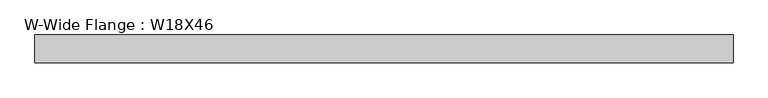
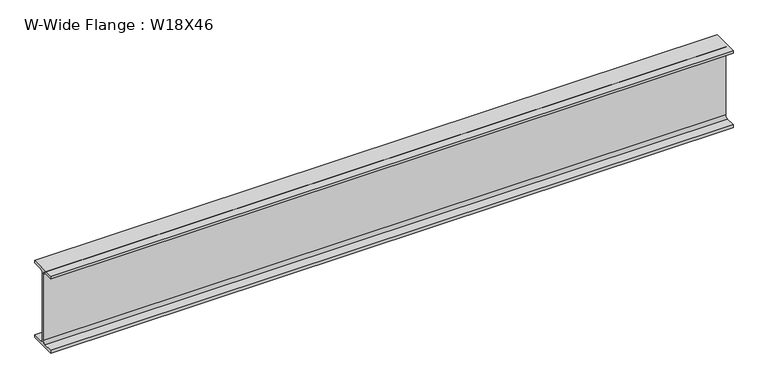
"""IFC4 building model written with IfcOpenShell, lengths in millimetres: beam geometry, W-Wide Flange : W18X46."""

from ifc_helpers import new_model, si_unit, point, frame, frame_2d, origin, place, context, project, spatial, polyline, circle_curve, trimmed, segment, composite_curve, outline, extrude, source, transform, mapped, element, save


def w_wide_flange_w18x46_e953a8c6(model_context):
    return source(origin(), model_context, "Body", "SweptSolid", [
        extrude(outline(composite_curve([segment(polyline([(76.962, -214.503), (76.962, -229.87), (-76.962, -229.87), (-76.962, -214.503), (-20.955, -214.503)]), True, "CONTINUOUS"), segment(trimmed(circle_curve(frame_2d((-20.955, -198.12)), 16.383), [point((-20.955, -214.503))], [point((-4.572, -198.12))], True, "CARTESIAN"), True, "CONTINUOUS"), segment(polyline([(-4.572, -198.12), (-4.572, 198.12)]), True, "CONTINUOUS"), segment(trimmed(circle_curve(frame_2d((-20.955, 198.12)), 16.383), [point((-4.572, 198.12))], [point((-20.955, 214.503))], True, "CARTESIAN"), True, "CONTINUOUS"), segment(polyline([(-20.955, 214.503), (-76.962, 214.503), (-76.962, 229.87), (76.962, 229.87), (76.962, 214.503), (20.955, 214.503)]), True, "CONTINUOUS"), segment(trimmed(circle_curve(frame_2d((20.955, 198.12)), 16.383), [point((20.955, 214.503))], [point((4.572, 198.12))], True, "CARTESIAN"), True, "CONTINUOUS"), segment(polyline([(4.572, 198.12), (4.572, -198.12)]), True, "CONTINUOUS"), segment(trimmed(circle_curve(frame_2d((20.955, -198.12)), 16.383), [point((4.572, -198.12))], [point((20.955, -214.503))], True, "CARTESIAN"), True, "CONTINUOUS"), segment(polyline([(20.955, -214.503), (76.962, -214.503)]), True, "CONTINUOUS")], self_intersect=False)), frame((-1916.1794068, 0.0, 0.0), z_axis=(1.0, 0.0, 0.0), x_axis=(0.0, 1.0, 0.0)), (0.0, 0.0, 1.0), 3852.9963136),
    ])


if __name__ == "__main__":
    model = new_model("IFC4")
    model_context = context("Model", 3, world=origin())
    ifc_project = project(units=[si_unit("LENGTHUNIT", "METRE", prefix="MILLI")], contexts=[model_context])
    site = spatial("IfcSite", under=ifc_project)
    building = spatial("IfcBuilding", under=site)
    placement = place(None, origin())
    w_wide_flange_w18x46_shape = w_wide_flange_w18x46_e953a8c6(model_context)
    element("IfcBeam", 1, ObjectType="W-Wide Flange : W18X46", at=placement, inside=building, context=model_context, shape_type="MappedRepresentation", body=[
        mapped(w_wide_flange_w18x46_shape, transform((0.0, 0.0, 0.0), x_axis=(1.0, 0.0, 0.0), y_axis=(0.0, 1.0, 0.0), z_axis=(0.0, 0.0, 1.0))),
    ])
    save(model, "model.ifc")

# Revit data of these elements
# Type "W-Wide Flange : W18X46"
#   Assembly Code = "B10"
#   W = 46
#   Length [instance default] = 5' - 0"
#   bf = 0' - 6.06"
#   d = 1' - 6.1"
#   k = 0' - 1 1/4"
#   k2 = 0' - 0.645"
#   tf = 0' - 0.605"
#   tw = 0' - 0.36"
#   A = 0.09375 SF
#   Structural Material [instance default] = Steel ASTM A992
# Element 1 (IfcBeam, "W-Wide Flange : W18X46")
#   Materials on its faces: "Steel ASTM A992"
# Materials
#   "Steel ASTM A992": class "Metal", colour RGB 199 199 199, transparency 0, Description = "Structural steel 50ksi", Cost = 0
